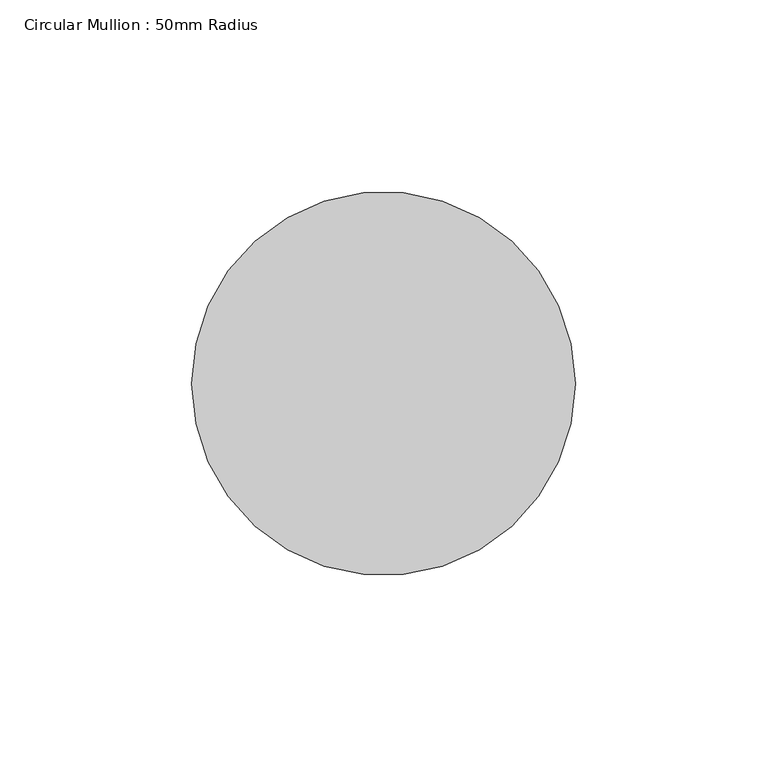
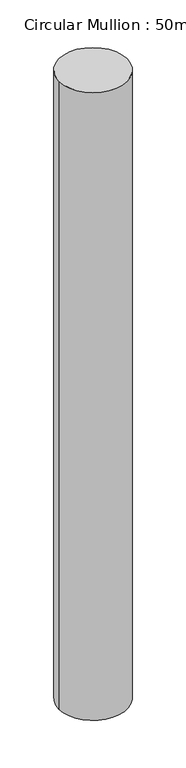
"""IFC4 building model written with IfcOpenShell, lengths in millimetres: member geometry, Circular Mullion : 50mm Radius."""

from ifc_helpers import new_model, si_unit, point, frame, origin, origin_2d, place, context, project, spatial, circle_curve, trimmed, segment, composite_curve, outline, extrude, source, transform, mapped, element, save


def circular_mullion_50mm_radius_1860f786(model_context):
    return source(origin(), model_context, "Body", "SweptSolid", [
        extrude(outline(composite_curve([segment(trimmed(circle_curve(origin_2d(), 50.0), [point((50.0, 0.0))], [point((-50.0, 0.0))], False, "CARTESIAN"), True, "CONTINUOUS"), segment(trimmed(circle_curve(origin_2d(), 50.0), [point((-50.0, 0.0))], [point((50.0, 0.0))], False, "CARTESIAN"), True, "CONTINUOUS")], self_intersect=False)), frame((0.0, 0.0, -975.1633517), z_axis=(0.0, 0.0, 1.0), x_axis=(1.0, 0.0, 0.0)), (0.0, 0.0, 1.0), 975.1633517),
    ])


if __name__ == "__main__":
    model = new_model("IFC4")
    model_context = context("Model", 3, world=origin())
    ifc_project = project(units=[si_unit("LENGTHUNIT", "METRE", prefix="MILLI")], contexts=[model_context])
    site = spatial("IfcSite", under=ifc_project)
    building = spatial("IfcBuilding", under=site)
    placement = place(None, origin())
    circular_mullion_50mm_radius_shape = circular_mullion_50mm_radius_1860f786(model_context)
    element("IfcMember", 1, ObjectType="Circular Mullion : 50mm Radius", at=placement, inside=building, context=model_context, shape_type="MappedRepresentation", body=[
        mapped(circular_mullion_50mm_radius_shape, transform((0.0, 0.0, 0.0), x_axis=(1.0, 0.0, 0.0), y_axis=(0.0, 1.0, 0.0), z_axis=(0.0, 0.0, 1.0))),
    ])
    save(model, "model.ifc")

# Revit data of these elements
# Type "Circular Mullion : 50mm Radius"
#   built-in parameter 1007350 = 0.164042 (stored number, unit not read)
# Element 1 (IfcMember, "Circular Mullion : 50mm Radius")
#   Materials on its faces: "Aluminium"
# Materials
#   "Aluminium": class "Metal", colour RGB 247 247 247, transparency 0, Description = "Aluminium 6061", Cost = 0
